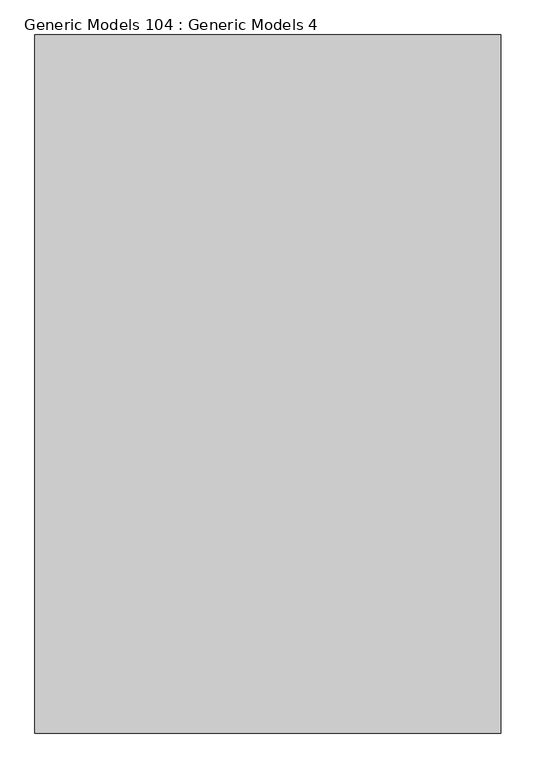
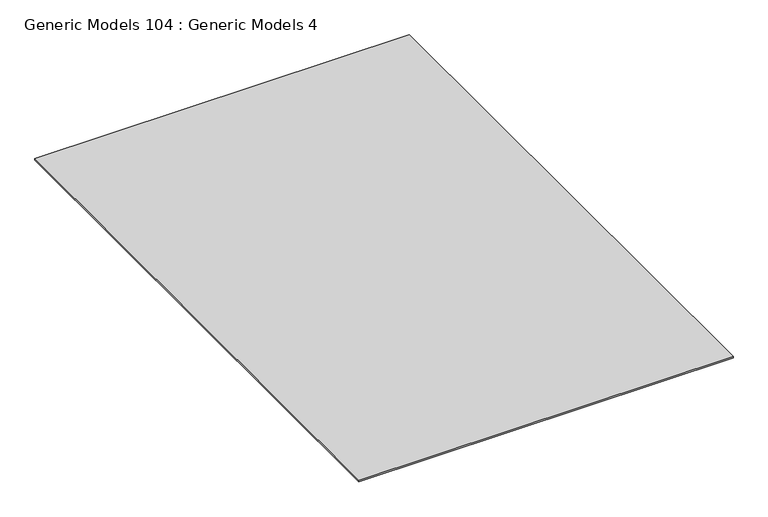
"""IFC4 building model written with IfcOpenShell, lengths in millimetres: proxy geometry, Generic Models 104 : Generic Models 4."""

from ifc_helpers import new_model, si_unit, frame, origin, place, context, project, spatial, polyline, outline, extrude, source, transform, mapped, element, save


def generic_models_104_generic_models_4_83a37be9(model_context):
    return source(origin(), model_context, "Body", "SweptSolid", [
        extrude(outline(polyline([(-2201.0836295, -6864.9230338), (-6470.8236296, -6864.9230338), (-6470.8236296, -464.1230338), (-2201.0836295, -464.1230338), (-2201.0836295, -6864.9230338)])), frame((0.0, 0.0, 126771.146), z_axis=(0.0, 0.0, 1.0), x_axis=(1.0, 0.0, 0.0)), (0.0, 0.0, 1.0), 19.05),
    ])


if __name__ == "__main__":
    model = new_model("IFC4")
    model_context = context("Model", 3, world=origin())
    ifc_project = project(units=[si_unit("LENGTHUNIT", "METRE", prefix="MILLI")], contexts=[model_context])
    site = spatial("IfcSite", under=ifc_project)
    building = spatial("IfcBuilding", under=site)
    placement = place(None, origin())
    generic_models_104_generic_models_4_shape = generic_models_104_generic_models_4_83a37be9(model_context)
    element("IfcBuildingElementProxy", 1, Name="Generic Models 104 : Generic Models 4", ObjectType="Generic Models 104 : Generic Models 4", at=placement, inside=building, context=model_context, shape_type="MappedRepresentation", body=[
        mapped(generic_models_104_generic_models_4_shape, transform((0.0, 0.0, 0.0), x_axis=(1.0, 0.0, 0.0), y_axis=(0.0, 1.0, 0.0), z_axis=(0.0, 0.0, 1.0))),
    ])
    save(model, "model.ifc")

# Revit data of these elements
# Element 1 (IfcBuildingElementProxy, "Generic Models 104 : Generic Models 4")
#   Materials on its faces: "_CDX PLYWOOD - SEE STRUCT DWGs"
# Materials
#   "_CDX PLYWOOD - SEE STRUCT DWGs": class "Generic", colour RGB 98 75 74, transparency 0, Cost = 0
